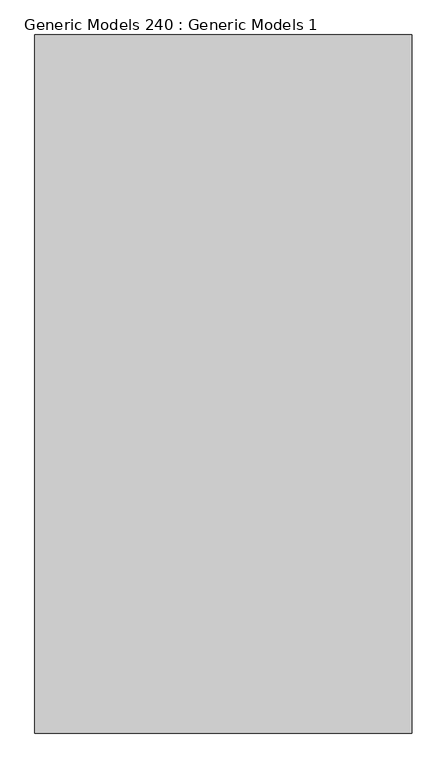
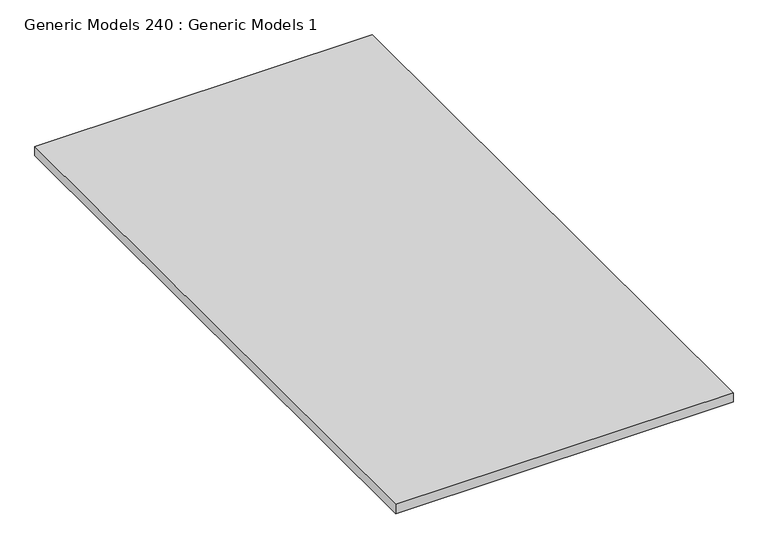
"""IFC4 building model written with IfcOpenShell, lengths in millimetres: proxy geometry, Generic Models 240 : Generic Models 1."""

import ifcopenshell
import ifcopenshell.guid

model = None  # the IFC model being written
_history = None  # IfcOwnerHistory: only IFC2X3 demands one
_inside = {}  # id of a spatial element -> (the spatial element, [elements in it])
_under = {}  # id of a project, library or spatial element -> (it, [spatial elements below it])
_declared = {}  # id of a project -> (the project, [libraries it declares])
_typed = {}  # id of a type object -> (the type object, [elements of that type])
_made_of = {}  # id of a material, layer set ... -> (it, [elements and type objects made of it])


def new_model(schema):
    """Start an empty IFC model of exactly this schema.

    Asked for "IFC4X3", IfcOpenShell would pick the latest addendum, in which some entities
    have other attributes; the version numbers below select the first issue.
    IFC2X3 requires an IfcOwnerHistory on every rooted entity: one is made here for all.
    """
    global model, _history
    if schema == "IFC4X3":
        model = ifcopenshell.file(schema_version=(4, 3, 0, 0))
    else:
        model = ifcopenshell.file(schema=schema)
    _inside.clear()
    _under.clear()
    _declared.clear()
    _typed.clear()
    _made_of.clear()
    _history = None
    if model.schema == "IFC2X3":
        org = make("IfcOrganization", Name="unknown")
        user = make(
            "IfcPersonAndOrganization",
            ThePerson=make("IfcPerson", FamilyName="unknown"),
            TheOrganization=org,
        )
        app = make(
            "IfcApplication",
            ApplicationDeveloper=org,
            Version="unknown",
            ApplicationFullName="unknown",
            ApplicationIdentifier="unknown",
        )
        _history = make(
            "IfcOwnerHistory",
            OwningUser=user,
            OwningApplication=app,
            ChangeAction="ADDED",
            CreationDate=0,
        )
    return model


def make(cls, **values):
    """One entity of the class cls with the attributes given. An attribute that is None is left unset."""
    return model.create_entity(
        cls, **{name: value for name, value in values.items() if value is not None}
    )


def rooted(cls, **values):
    """An entity with a GlobalId (a new one), such as an element, a storey or a relation."""
    return make(cls, GlobalId=ifcopenshell.guid.new(), OwnerHistory=_history, **values)


def si_unit(unit_type, name, prefix=None):
    """IfcSIUnit, for example si_unit("LENGTHUNIT", "METRE", prefix="MILLI")."""
    return make("IfcSIUnit", UnitType=unit_type, Prefix=prefix, Name=name)


def assignment(units):
    """IfcUnitAssignment: the units of a project."""
    return None if units is None else make("IfcUnitAssignment", Units=units)


def point(xyz):
    """IfcCartesianPoint."""
    return None if xyz is None else make("IfcCartesianPoint", Coordinates=xyz)


def direction(xyz):
    """IfcDirection."""
    return None if xyz is None else make("IfcDirection", DirectionRatios=xyz)


def frame(location, z_axis=None, x_axis=None):
    """IfcAxis2Placement3D, a coordinate frame: its origin and axes. An axis left out is left unset."""
    return make(
        "IfcAxis2Placement3D",
        Location=point(location),
        Axis=direction(z_axis),
        RefDirection=direction(x_axis),
    )


def origin():
    """The frame at (0, 0, 0) with its axes left unset."""
    return frame((0.0, 0.0, 0.0))


def place(relative_to, where):
    """IfcLocalPlacement: puts the frame where relative to a parent placement (None: the world)."""
    return make(
        "IfcLocalPlacement", PlacementRelTo=relative_to, RelativePlacement=where
    )


def context(
    kind, dimensions, precision=None, world=None, true_north=None, identifier=None
):
    """IfcGeometricRepresentationContext, for example the 3D "Model" context."""
    return make(
        "IfcGeometricRepresentationContext",
        ContextIdentifier=identifier,
        ContextType=kind,
        CoordinateSpaceDimension=dimensions,
        Precision=precision,
        WorldCoordinateSystem=world,
        TrueNorth=true_north,
    )


def project(units=None, contexts=None):
    """IfcProject with its units and contexts."""
    return rooted(
        "IfcProject",
        Name="project",
        RepresentationContexts=contexts,
        UnitsInContext=assignment(units),
    )


def spatial(cls, under=None, at=None, **own):
    """A site, building, storey or space (cls), placed at a placement, below another one or the project."""
    s = rooted(cls, ObjectPlacement=at, **own)
    if under is not None:
        _under.setdefault(under.id(), (under, []))[1].append(s)
    return s


def polyline(points):
    """IfcPolyline through the points."""
    return make("IfcPolyline", Points=[point(p) for p in points])


def outline(outer, holes=None, kind="AREA"):
    """IfcArbitraryClosedProfileDef: a profile drawn as a closed curve; with holes, ...WithVoids."""
    if holes is None:
        return make("IfcArbitraryClosedProfileDef", ProfileType=kind, OuterCurve=outer)
    return make(
        "IfcArbitraryProfileDefWithVoids",
        ProfileType=kind,
        OuterCurve=outer,
        InnerCurves=holes,
    )


def extrude(swept, where, along, depth):
    """IfcExtrudedAreaSolid: the profile swept, set in the frame where, extruded along a direction by depth."""
    return make(
        "IfcExtrudedAreaSolid",
        SweptArea=swept,
        Position=where,
        ExtrudedDirection=direction(along),
        Depth=depth,
    )


def shape(context_of_items, identifier, shape_type, items):
    """IfcShapeRepresentation: the items that make up one representation, for example the "Body"."""
    return make(
        "IfcShapeRepresentation",
        ContextOfItems=context_of_items,
        RepresentationIdentifier=identifier,
        RepresentationType=shape_type,
        Items=items,
    )


def source(mapping_origin, context_of_items, identifier, shape_type, items):
    """IfcRepresentationMap: a shape defined once, which mapped items show again and again."""
    return make(
        "IfcRepresentationMap",
        MappingOrigin=mapping_origin,
        MappedRepresentation=shape(context_of_items, identifier, shape_type, items),
    )


def transform(
    local_origin,
    x_axis=None,
    y_axis=None,
    z_axis=None,
    scale=None,
    scale2=None,
    scale3=None,
    uniform=True,
):
    """IfcCartesianTransformationOperator3D, or its non-uniform kind. x_axis, y_axis, z_axis: its Axis1, 2, 3."""
    if uniform:
        return make(
            "IfcCartesianTransformationOperator3D",
            Axis1=direction(x_axis),
            Axis2=direction(y_axis),
            LocalOrigin=point(local_origin),
            Scale=scale,
            Axis3=direction(z_axis),
        )
    return make(
        "IfcCartesianTransformationOperator3DnonUniform",
        Axis1=direction(x_axis),
        Axis2=direction(y_axis),
        LocalOrigin=point(local_origin),
        Scale=scale,
        Axis3=direction(z_axis),
        Scale2=scale2,
        Scale3=scale3,
    )


def mapped(mapping_source, mapping_target):
    """IfcMappedItem: shows the shape of a source again, moved by a transform."""
    return make(
        "IfcMappedItem", MappingSource=mapping_source, MappingTarget=mapping_target
    )


def made_of(thing, what):
    """Note that an element or type object is made of a material, layer set ...; save() writes the relation."""
    if what is not None:
        _made_of.setdefault(what.id(), (what, []))[1].append(thing)
    return thing


def element(
    cls,
    number,
    at=None,
    inside=None,
    cuts=None,
    type_object=None,
    material=None,
    context=None,
    identifier="Body",
    shape_type=None,
    held_by="IfcProductDefinitionShape",
    body=None,
    shapes=None,
    **own,
):
    """One element of the class cls, such as IfcWall. Its Tag is "e" and its number.

    at: its placement. inside: the storey or other place that contains it. cuts: it is an
    opening in that element (IfcRelVoidsElement). A single representation is given by context,
    identifier, shape_type and body (its items); several are given by shapes. held_by: the class
    of the entity that holds the representations. save() writes the other relations.
    """
    e = rooted(cls, Tag="e%d" % number, ObjectPlacement=at, **own)
    if body is not None:
        shapes = [shape(context, identifier, shape_type, body)]
    if shapes is not None:
        e.Representation = make(held_by, Representations=shapes)
    if inside is not None:
        _inside.setdefault(inside.id(), (inside, []))[1].append(e)
    if cuts is not None:
        rooted(
            "IfcRelVoidsElement", RelatingBuildingElement=cuts, RelatedOpeningElement=e
        )
    if type_object is not None:
        _typed.setdefault(type_object.id(), (type_object, []))[1].append(e)
    return made_of(e, material)


def aggregate(whole, parts):
    """IfcRelAggregates: a whole, such as a stair, and the parts it consists of."""
    return rooted("IfcRelAggregates", RelatingObject=whole, RelatedObjects=parts)


def save(model, path):
    """Write the relations noted so far, then the file.

    IfcRelAggregates (storeys below a building ...), IfcRelContainedInSpatialStructure (elements
    in a storey), IfcRelDefinesByType, IfcRelAssociatesMaterial and IfcRelDeclares: one each for
    every whole, place, type object, material and project.
    """
    for whole, parts in _under.values():
        aggregate(whole, parts)
    for where, things in _inside.values():
        rooted(
            "IfcRelContainedInSpatialStructure",
            RelatedElements=things,
            RelatingStructure=where,
        )
    for kind, things in _typed.values():
        rooted("IfcRelDefinesByType", RelatedObjects=things, RelatingType=kind)
    for what, things in _made_of.values():
        rooted("IfcRelAssociatesMaterial", RelatedObjects=things, RelatingMaterial=what)
    for by, libraries in _declared.values():
        rooted("IfcRelDeclares", RelatingContext=by, RelatedDefinitions=libraries)
    model.write(path)


def generic_models_240_generic_models_1_611786cf(model_context):
    return source(origin(), model_context, "Body", "SweptSolid", [
        extrude(outline(polyline([(49128.3625, 1219.2), (49128.3625, 0.0), (48469.55, 0.0), (48469.55, 1219.2), (49128.3625, 1219.2)])), frame((0.0, 0.0, 5649.9125), z_axis=(0.0, 0.0, 1.0), x_axis=(1.0, 0.0, 0.0)), (0.0, 0.0, 1.0), 19.05),
    ])


if __name__ == "__main__":
    model = new_model("IFC4")
    model_context = context("Model", 3, world=origin())
    ifc_project = project(units=[si_unit("LENGTHUNIT", "METRE", prefix="MILLI")], contexts=[model_context])
    site = spatial("IfcSite", under=ifc_project)
    building = spatial("IfcBuilding", under=site)
    placement = place(None, origin())
    generic_models_240_generic_models_1_shape = generic_models_240_generic_models_1_611786cf(model_context)
    element("IfcBuildingElementProxy", 1, Name="Generic Models 240 : Generic Models 1", ObjectType="Generic Models 240 : Generic Models 1", at=placement, inside=building, context=model_context, shape_type="MappedRepresentation", body=[
        mapped(generic_models_240_generic_models_1_shape, transform((0.0, 0.0, 0.0), x_axis=(1.0, 0.0, 0.0), y_axis=(0.0, 1.0, 0.0), z_axis=(0.0, 0.0, 1.0))),
    ])
    save(model, "model.ifc")

# Revit data of these elements
# Element 1 (IfcBuildingElementProxy, "Generic Models 240 : Generic Models 1")
#   Materials on its faces: "EXISTING SUBSTRATE"
# Materials
#   "EXISTING SUBSTRATE": class "Unassigned", colour RGB 196 177 123, transparency 0, Cost = 0
